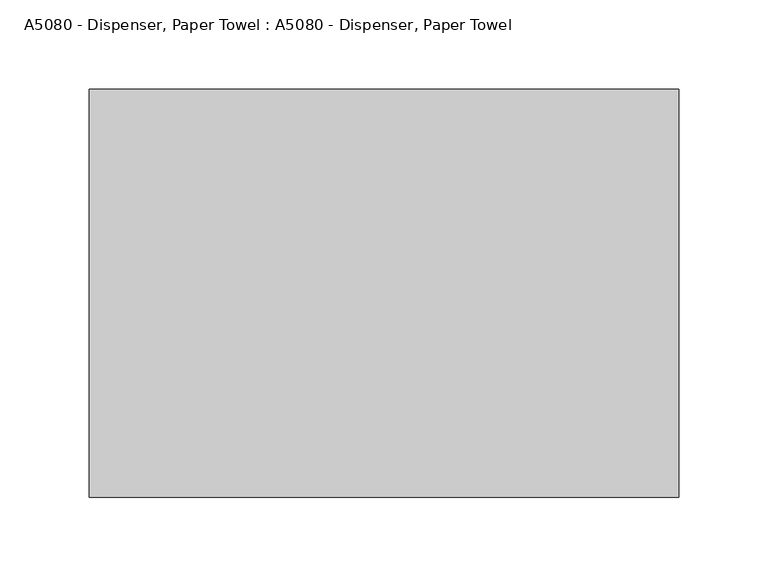
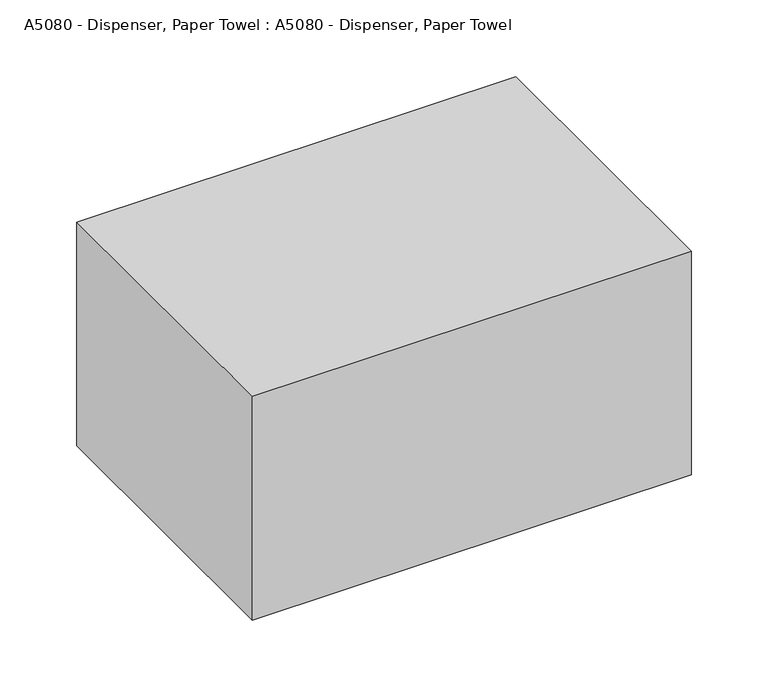
"""IFC4 building model written with IfcOpenShell, lengths in millimetres: proxy geometry, A5080 - Dispenser, Paper Towel : A5080 - Dispenser, Paper Towel."""

import ifcopenshell
import ifcopenshell.guid

model = None  # the IFC model being written
_history = None  # IfcOwnerHistory: only IFC2X3 demands one
_inside = {}  # id of a spatial element -> (the spatial element, [elements in it])
_under = {}  # id of a project, library or spatial element -> (it, [spatial elements below it])
_declared = {}  # id of a project -> (the project, [libraries it declares])
_typed = {}  # id of a type object -> (the type object, [elements of that type])
_made_of = {}  # id of a material, layer set ... -> (it, [elements and type objects made of it])


def new_model(schema):
    """Start an empty IFC model of exactly this schema.

    Asked for "IFC4X3", IfcOpenShell would pick the latest addendum, in which some entities
    have other attributes; the version numbers below select the first issue.
    IFC2X3 requires an IfcOwnerHistory on every rooted entity: one is made here for all.
    """
    global model, _history
    if schema == "IFC4X3":
        model = ifcopenshell.file(schema_version=(4, 3, 0, 0))
    else:
        model = ifcopenshell.file(schema=schema)
    _inside.clear()
    _under.clear()
    _declared.clear()
    _typed.clear()
    _made_of.clear()
    _history = None
    if model.schema == "IFC2X3":
        org = make("IfcOrganization", Name="unknown")
        user = make(
            "IfcPersonAndOrganization",
            ThePerson=make("IfcPerson", FamilyName="unknown"),
            TheOrganization=org,
        )
        app = make(
            "IfcApplication",
            ApplicationDeveloper=org,
            Version="unknown",
            ApplicationFullName="unknown",
            ApplicationIdentifier="unknown",
        )
        _history = make(
            "IfcOwnerHistory",
            OwningUser=user,
            OwningApplication=app,
            ChangeAction="ADDED",
            CreationDate=0,
        )
    return model


def make(cls, **values):
    """One entity of the class cls with the attributes given. An attribute that is None is left unset."""
    return model.create_entity(
        cls, **{name: value for name, value in values.items() if value is not None}
    )


def rooted(cls, **values):
    """An entity with a GlobalId (a new one), such as an element, a storey or a relation."""
    return make(cls, GlobalId=ifcopenshell.guid.new(), OwnerHistory=_history, **values)


def si_unit(unit_type, name, prefix=None):
    """IfcSIUnit, for example si_unit("LENGTHUNIT", "METRE", prefix="MILLI")."""
    return make("IfcSIUnit", UnitType=unit_type, Prefix=prefix, Name=name)


def assignment(units):
    """IfcUnitAssignment: the units of a project."""
    return None if units is None else make("IfcUnitAssignment", Units=units)


def point(xyz):
    """IfcCartesianPoint."""
    return None if xyz is None else make("IfcCartesianPoint", Coordinates=xyz)


def direction(xyz):
    """IfcDirection."""
    return None if xyz is None else make("IfcDirection", DirectionRatios=xyz)


def frame(location, z_axis=None, x_axis=None):
    """IfcAxis2Placement3D, a coordinate frame: its origin and axes. An axis left out is left unset."""
    return make(
        "IfcAxis2Placement3D",
        Location=point(location),
        Axis=direction(z_axis),
        RefDirection=direction(x_axis),
    )


def origin():
    """The frame at (0, 0, 0) with its axes left unset."""
    return frame((0.0, 0.0, 0.0))


def origin_with_axes():
    """The frame at (0, 0, 0) with the z axis (0, 0, 1) and the x axis (1, 0, 0) written out."""
    return frame((0.0, 0.0, 0.0), z_axis=(0.0, 0.0, 1.0), x_axis=(1.0, 0.0, 0.0))


def place(relative_to, where):
    """IfcLocalPlacement: puts the frame where relative to a parent placement (None: the world)."""
    return make(
        "IfcLocalPlacement", PlacementRelTo=relative_to, RelativePlacement=where
    )


def context(
    kind, dimensions, precision=None, world=None, true_north=None, identifier=None
):
    """IfcGeometricRepresentationContext, for example the 3D "Model" context."""
    return make(
        "IfcGeometricRepresentationContext",
        ContextIdentifier=identifier,
        ContextType=kind,
        CoordinateSpaceDimension=dimensions,
        Precision=precision,
        WorldCoordinateSystem=world,
        TrueNorth=true_north,
    )


def project(units=None, contexts=None):
    """IfcProject with its units and contexts."""
    return rooted(
        "IfcProject",
        Name="project",
        RepresentationContexts=contexts,
        UnitsInContext=assignment(units),
    )


def spatial(cls, under=None, at=None, **own):
    """A site, building, storey or space (cls), placed at a placement, below another one or the project."""
    s = rooted(cls, ObjectPlacement=at, **own)
    if under is not None:
        _under.setdefault(under.id(), (under, []))[1].append(s)
    return s


def polyline(points):
    """IfcPolyline through the points."""
    return make("IfcPolyline", Points=[point(p) for p in points])


def outline(outer, holes=None, kind="AREA"):
    """IfcArbitraryClosedProfileDef: a profile drawn as a closed curve; with holes, ...WithVoids."""
    if holes is None:
        return make("IfcArbitraryClosedProfileDef", ProfileType=kind, OuterCurve=outer)
    return make(
        "IfcArbitraryProfileDefWithVoids",
        ProfileType=kind,
        OuterCurve=outer,
        InnerCurves=holes,
    )


def extrude(swept, where, along, depth):
    """IfcExtrudedAreaSolid: the profile swept, set in the frame where, extruded along a direction by depth."""
    return make(
        "IfcExtrudedAreaSolid",
        SweptArea=swept,
        Position=where,
        ExtrudedDirection=direction(along),
        Depth=depth,
    )


def shape(context_of_items, identifier, shape_type, items):
    """IfcShapeRepresentation: the items that make up one representation, for example the "Body"."""
    return make(
        "IfcShapeRepresentation",
        ContextOfItems=context_of_items,
        RepresentationIdentifier=identifier,
        RepresentationType=shape_type,
        Items=items,
    )


def source(mapping_origin, context_of_items, identifier, shape_type, items):
    """IfcRepresentationMap: a shape defined once, which mapped items show again and again."""
    return make(
        "IfcRepresentationMap",
        MappingOrigin=mapping_origin,
        MappedRepresentation=shape(context_of_items, identifier, shape_type, items),
    )


def transform(
    local_origin,
    x_axis=None,
    y_axis=None,
    z_axis=None,
    scale=None,
    scale2=None,
    scale3=None,
    uniform=True,
):
    """IfcCartesianTransformationOperator3D, or its non-uniform kind. x_axis, y_axis, z_axis: its Axis1, 2, 3."""
    if uniform:
        return make(
            "IfcCartesianTransformationOperator3D",
            Axis1=direction(x_axis),
            Axis2=direction(y_axis),
            LocalOrigin=point(local_origin),
            Scale=scale,
            Axis3=direction(z_axis),
        )
    return make(
        "IfcCartesianTransformationOperator3DnonUniform",
        Axis1=direction(x_axis),
        Axis2=direction(y_axis),
        LocalOrigin=point(local_origin),
        Scale=scale,
        Axis3=direction(z_axis),
        Scale2=scale2,
        Scale3=scale3,
    )


def mapped(mapping_source, mapping_target):
    """IfcMappedItem: shows the shape of a source again, moved by a transform."""
    return make(
        "IfcMappedItem", MappingSource=mapping_source, MappingTarget=mapping_target
    )


def made_of(thing, what):
    """Note that an element or type object is made of a material, layer set ...; save() writes the relation."""
    if what is not None:
        _made_of.setdefault(what.id(), (what, []))[1].append(thing)
    return thing


def element(
    cls,
    number,
    at=None,
    inside=None,
    cuts=None,
    type_object=None,
    material=None,
    context=None,
    identifier="Body",
    shape_type=None,
    held_by="IfcProductDefinitionShape",
    body=None,
    shapes=None,
    **own,
):
    """One element of the class cls, such as IfcWall. Its Tag is "e" and its number.

    at: its placement. inside: the storey or other place that contains it. cuts: it is an
    opening in that element (IfcRelVoidsElement). A single representation is given by context,
    identifier, shape_type and body (its items); several are given by shapes. held_by: the class
    of the entity that holds the representations. save() writes the other relations.
    """
    e = rooted(cls, Tag="e%d" % number, ObjectPlacement=at, **own)
    if body is not None:
        shapes = [shape(context, identifier, shape_type, body)]
    if shapes is not None:
        e.Representation = make(held_by, Representations=shapes)
    if inside is not None:
        _inside.setdefault(inside.id(), (inside, []))[1].append(e)
    if cuts is not None:
        rooted(
            "IfcRelVoidsElement", RelatingBuildingElement=cuts, RelatedOpeningElement=e
        )
    if type_object is not None:
        _typed.setdefault(type_object.id(), (type_object, []))[1].append(e)
    return made_of(e, material)


def aggregate(whole, parts):
    """IfcRelAggregates: a whole, such as a stair, and the parts it consists of."""
    return rooted("IfcRelAggregates", RelatingObject=whole, RelatedObjects=parts)


def save(model, path):
    """Write the relations noted so far, then the file.

    IfcRelAggregates (storeys below a building ...), IfcRelContainedInSpatialStructure (elements
    in a storey), IfcRelDefinesByType, IfcRelAssociatesMaterial and IfcRelDeclares: one each for
    every whole, place, type object, material and project.
    """
    for whole, parts in _under.values():
        aggregate(whole, parts)
    for where, things in _inside.values():
        rooted(
            "IfcRelContainedInSpatialStructure",
            RelatedElements=things,
            RelatingStructure=where,
        )
    for kind, things in _typed.values():
        rooted("IfcRelDefinesByType", RelatedObjects=things, RelatingType=kind)
    for what, things in _made_of.values():
        rooted("IfcRelAssociatesMaterial", RelatedObjects=things, RelatingMaterial=what)
    for by, libraries in _declared.values():
        rooted("IfcRelDeclares", RelatingContext=by, RelatedDefinitions=libraries)
    model.write(path)


def a5080_dispenser_paper_towel_a5080_dispenser_paper_towel_604ea92f(model_context):
    return source(origin(), model_context, "Body", "SweptSolid", [
        extrude(outline(polyline([(165.1, -228.6), (-165.1, -228.6), (-165.1, 0.0), (165.1, 0.0), (165.1, -228.6)])), origin_with_axes(), (0.0, 0.0, 1.0), 177.8),
        extrude(outline(polyline([(-165.1, -228.6), (-165.1, 0.0), (165.1, 0.0), (165.1, -228.6), (-165.1, -228.6)])), origin_with_axes(), (0.0, 0.0, 1.0), 177.8),
    ])


if __name__ == "__main__":
    model = new_model("IFC4")
    model_context = context("Model", 3, world=origin())
    ifc_project = project(units=[si_unit("LENGTHUNIT", "METRE", prefix="MILLI")], contexts=[model_context])
    site = spatial("IfcSite", under=ifc_project)
    building = spatial("IfcBuilding", under=site)
    placement = place(None, origin())
    a5080_dispenser_paper_towel_a5080_dispenser_paper_towel_shape = a5080_dispenser_paper_towel_a5080_dispenser_paper_towel_604ea92f(model_context)
    element("IfcBuildingElementProxy", 1, Name="A5080 - Dispenser, Paper Towel : A5080 - Dispenser, Paper Towel", ObjectType="A5080 - Dispenser, Paper Towel : A5080 - Dispenser, Paper Towel", at=placement, inside=building, context=model_context, shape_type="MappedRepresentation", body=[
        mapped(a5080_dispenser_paper_towel_a5080_dispenser_paper_towel_shape, transform((0.0, 0.0, 0.0), x_axis=(1.0, 0.0, 0.0), y_axis=(0.0, 1.0, 0.0), z_axis=(0.0, 0.0, 1.0))),
    ])
    save(model, "model.ifc")

# Revit data of these elements
# Type "A5080 - Dispenser, Paper Towel : A5080 - Dispenser, Paper Towel"
#   Watts2 = "0"
#   Watts1 = "0"
#   Unit_Issue = "EA"
#   UTIL_6_Misc = "-"
#   UTIL_5_NonMedGas = "-"
#   UTIL_4_MiscGas = "-"
#   UTIL_3_MedGas = "-"
#   UTIL_2_Elec = "-"
#   UTIL_1_WaterDrain = "-"
#   Nomenclature = "Dispenser, Paper Towel, SS, Surface Mounted"
#   NSN = "4510"
#   Location [instance default] = ""
#   JSN = "A5080"
#   Fund_Source_VA = "-"
#   Fund_Source_Navy = "-"
#   Fund_Source_Army = "-"
#   Fund_Source_AF = "-"
#   ELEC_Volts2 = "0"
#   ELEC_Volts1 = "0"
#   ELEC_Phase2 = "0"
#   ELEC_Phase1 = "0"
#   ELEC_HertzSwitch = "0"
#   ELEC_HertzDependent = "0"
#   ELEC_Hertz = "0"
#   ELEC_Amps2 = "0"
#   ELEC_Amps1 = "0"
#   DetailDescription = "A surface mounted, satin finish stainless steel, single-fold, paper towel dispenser. Dispenser features: tumbler lock; front hinged at bottom; and refill indicator slot. Minimum capacity 400 single-fold paper towels. For general purpose use throughout the facility."
#   CAT_VA = "A"
#   CAT_Navy = "A"
#   CAT_IHS = "-"
#   CAT_Army = "A"
#   CAT_AF = "A"
#   BTUperhour = "0"
#   Weight_IP = 4
#   Default Elevation = 4' - 0"
#   DIM_Width_IP = 1' - 1"
#   DIM_Height_IP = 0' - 9"
#   DIM_Depth_IP = 0' - 7"
#   Assembly Code = ""
# Element 1 (IfcBuildingElementProxy, "A5080 - Dispenser, Paper Towel : A5080 - Dispenser, Paper Towel")
#   Location = "UCCL2"
#   Materials on its faces: "EquipSpace", "Wall Material (1)"
# Materials
#   "EquipSpace": class "Unassigned", colour RGB 221 217 195, transparency 0.5
#   "Wall Material (1)": class "Miscellaneous", colour RGB 234 233 232, transparency 0
